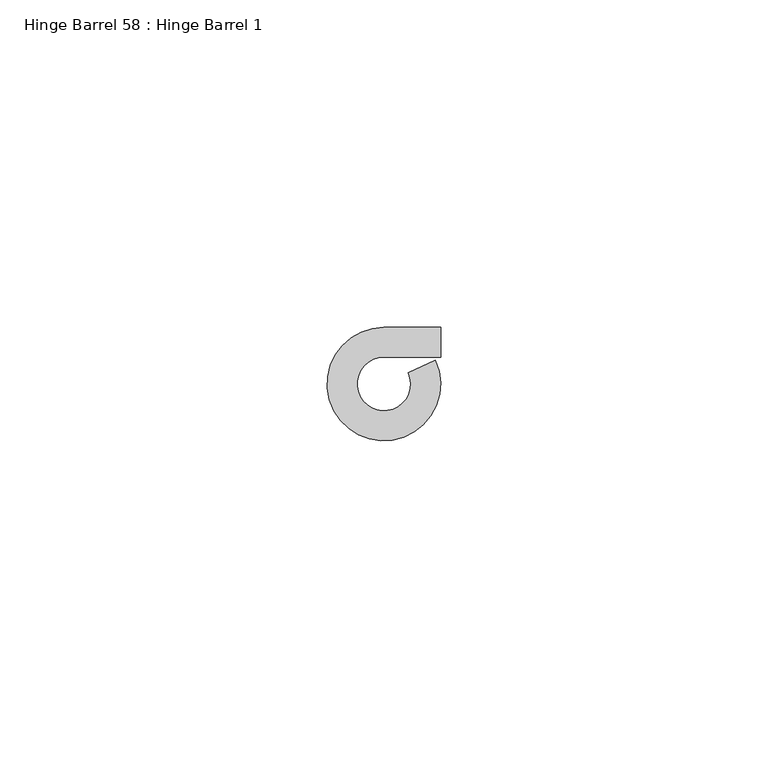
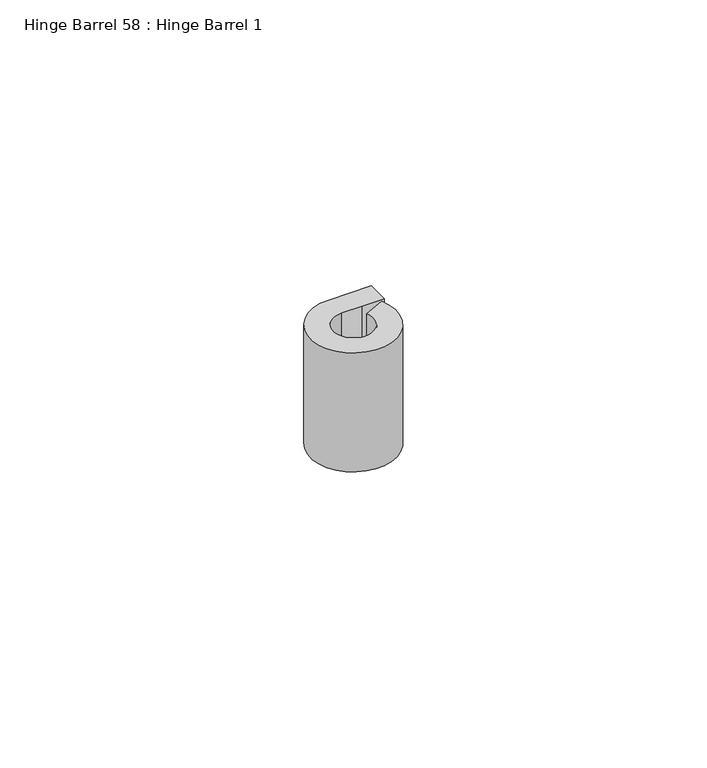
"""IFC4 building model written with IfcOpenShell, lengths in millimetres: proxy geometry, Hinge Barrel 58 : Hinge Barrel 1."""

from ifc_helpers import new_model, si_unit, point, frame, frame_2d, origin, place, context, project, spatial, polyline, circle_curve, trimmed, segment, composite_curve, outline, extrude, source, transform, mapped, element, save


def hinge_barrel_58_hinge_barrel_1_8e11106c(model_context):
    return source(origin(), model_context, "Body", "SweptSolid", [
        extrude(outline(composite_curve([segment(polyline([(587323.2214739, -536306.2758841), (587319.1320739, -536306.2758841)]), True, "CONTINUOUS"), segment(trimmed(circle_curve(frame_2d((587319.1320739, -536310.3652841)), 4.0894), [point((587319.1320739, -536306.2758841))], [point((587322.8436736, -536308.6485371))], True, "CARTESIAN"), True, "CONTINUOUS"), segment(polyline([(587322.8436736, -536308.6485371), (587326.986084, -536306.7325249)]), True, "CONTINUOUS"), segment(trimmed(circle_curve(frame_2d((587319.1320739, -536310.3652841)), 8.6534625), [point((587326.986084, -536306.7325249))], [point((587319.1320739, -536301.7118216))], False, "CARTESIAN"), True, "CONTINUOUS"), segment(polyline([(587319.1320739, -536301.7118216), (587327.7934739, -536301.7118216), (587327.7934739, -536306.2758841), (587323.2214739, -536306.2758841)]), True, "CONTINUOUS")], self_intersect=False)), frame((0.0, 0.0, 412.75), z_axis=(0.0, 0.0, 1.0), x_axis=(1.0, 0.0, 0.0)), (0.0, 0.0, 1.0), 25.4),
    ])


if __name__ == "__main__":
    model = new_model("IFC4")
    model_context = context("Model", 3, world=origin())
    ifc_project = project(units=[si_unit("LENGTHUNIT", "METRE", prefix="MILLI")], contexts=[model_context])
    site = spatial("IfcSite", under=ifc_project)
    building = spatial("IfcBuilding", under=site)
    placement = place(None, origin())
    hinge_barrel_58_hinge_barrel_1_shape = hinge_barrel_58_hinge_barrel_1_8e11106c(model_context)
    element("IfcBuildingElementProxy", 1, Name="Hinge Barrel 58 : Hinge Barrel 1", ObjectType="Hinge Barrel 58 : Hinge Barrel 1", at=placement, inside=building, context=model_context, shape_type="MappedRepresentation", body=[
        mapped(hinge_barrel_58_hinge_barrel_1_shape, transform((0.0, 0.0, 0.0), x_axis=(1.0, 0.0, 0.0), y_axis=(0.0, 1.0, 0.0), z_axis=(0.0, 0.0, 1.0))),
    ])
    save(model, "model.ifc")

# Revit data of these elements
# Element 1 (IfcBuildingElementProxy, "Hinge Barrel 58 : Hinge Barrel 1")
#   Materials on its faces: "6\"X6\" WELD-ON STL BUTT HINGE"
# Materials
#   "6\"X6\" WELD-ON STL BUTT HINGE": class "Metal", colour RGB 189 187 185, transparency 0, Description = "Carbon steel", Cost = 0
